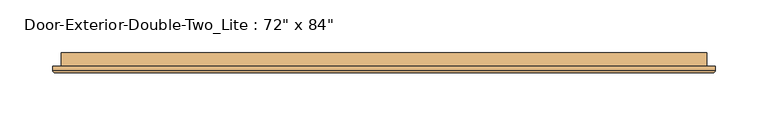
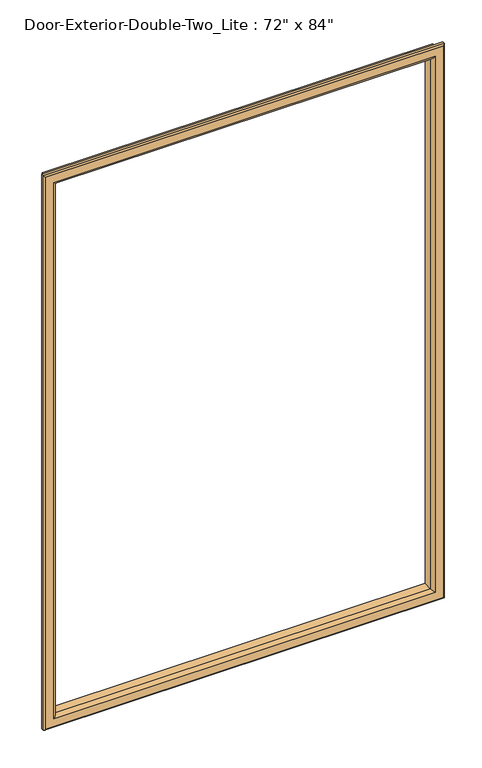
"""IFC4 building model written with IfcOpenShell, lengths in millimetres: door geometry."""

from ifc_helpers import new_model, si_unit, frame, origin, place, context, project, spatial, ellipse_curve, source, transform, mapped, element, save
from ifc_brep_helpers import plane_surface, cylinder_surface, advanced_brep


def door_d0d74375(model_context):
    return source(origin(), model_context, "Body", "AdvancedBrep", [
        advanced_brep(
        [(-762.0, 36.5125, 1117.6), (-762.0, 23.8125, 1117.6), (-762.0, 23.8125, 2016.125), (-762.0, 36.5125, 2016.125), (-750.0, 22.8125, 1129.6), (-750.0, 36.5125, 1129.6), (-750.0, 36.5125, 2004.125), (-750.0, 22.8125, 2004.125), (-755.0, 17.8125, 1124.6), (-755.0, 17.8125, 2009.125), (-770.0, 19.8125, 1109.6), (-768.0, 17.8125, 1111.6), (-768.0, 17.8125, 2022.125), (-770.0, 19.8125, 2024.125), (-770.0, 23.8125, 1109.6), (-770.0, 23.8125, 2024.125), (-152.4, 23.8125, 2016.125), (-152.4, 36.5125, 2016.125), (-164.4, 36.5125, 2004.125), (-164.4, 22.8125, 2004.125), (-159.4, 17.8125, 2009.125), (-146.4, 17.8125, 2022.125), (-144.4, 19.8125, 2024.125), (-144.4, 23.8125, 2024.125), (-152.4, 23.8125, 1117.6), (-152.4, 36.5125, 1117.6), (-164.4, 36.5125, 1129.6), (-164.4, 22.8125, 1129.6), (-159.4, 17.8125, 1124.6), (-146.4, 17.8125, 1111.6), (-144.4, 19.8125, 1109.6), (-144.4, 23.8125, 1109.6)],
        [
            (0, 1),
            (1, 2),
            (2, 3),
            (3, 0),
            (4, 5),
            (5, 6),
            (6, 7),
            (7, 4),
            (8, 4, ellipse_curve(frame((-755.0, 22.8125, 1124.6), z_axis=(-0.7071067811865475, 0.0, 0.7071067811865475), x_axis=(-0.7071067811865474, 0.0, -0.7071067811865476)), 7.0710678, 5.0)),
            (7, 9, ellipse_curve(frame((-755.0, 22.8125, 2009.125), z_axis=(-0.7071067811865475, 0.0, -0.7071067811865475), x_axis=(0.7071067811865474, 0.0, -0.7071067811865476)), 7.0710678, 5.0)),
            (9, 8),
            (10, 11, ellipse_curve(frame((-768.0, 19.8125, 1111.6), z_axis=(-0.7071067811865475, 0.0, 0.7071067811865475), x_axis=(-0.7071067811865474, 0.0, -0.7071067811865476)), 2.8284271, 2.0)),
            (11, 12),
            (12, 13, ellipse_curve(frame((-768.0, 19.8125, 2022.125), z_axis=(-0.7071067811865475, 0.0, -0.7071067811865475), x_axis=(0.7071067811865474, 0.0, -0.7071067811865476)), 2.8284271, 2.0)),
            (13, 10),
            (14, 10),
            (13, 15),
            (15, 14),
            (2, 16),
            (16, 17),
            (17, 3),
            (6, 18),
            (18, 19),
            (19, 7),
            (19, 20, ellipse_curve(frame((-159.4, 22.8125, 2009.125), z_axis=(-0.7071067811865475, 0.0, 0.7071067811865475), x_axis=(-0.7071067811865476, 0.0, -0.7071067811865474)), 7.0710678, 5.0)),
            (20, 9),
            (12, 21),
            (21, 22, ellipse_curve(frame((-146.4, 19.8125, 2022.125), z_axis=(-0.7071067811865475, 0.0, 0.7071067811865475), x_axis=(-0.7071067811865476, 0.0, -0.7071067811865474)), 2.8284271, 2.0)),
            (22, 13),
            (22, 23),
            (23, 15),
            (16, 24),
            (24, 25),
            (25, 17),
            (18, 26),
            (26, 27),
            (27, 19),
            (27, 28, ellipse_curve(frame((-159.4, 22.8125, 1124.6), z_axis=(0.7071067811865475, 0.0, 0.7071067811865475), x_axis=(-0.7071067811865474, 0.0, 0.7071067811865476)), 7.0710678, 5.0)),
            (28, 20),
            (21, 29),
            (29, 30, ellipse_curve(frame((-146.4, 19.8125, 1111.6), z_axis=(0.7071067811865475, 0.0, 0.7071067811865475), x_axis=(-0.7071067811865474, 0.0, 0.7071067811865476)), 2.8284271, 2.0)),
            (30, 22),
            (30, 31),
            (31, 23),
            (31, 14),
            (1, 24),
            (0, 25),
            (5, 26),
            (4, 27),
            (8, 28),
            (11, 29),
            (10, 30),
        ],
        [
            plane_surface(frame((-762.0, 23.8125, 1117.6), z_axis=(-1.0, 0.0, 0.0), x_axis=(0.0, 0.0, 1.0))),
            plane_surface(frame((-750.0, 36.5125, 1129.6), z_axis=(1.0, 0.0, 0.0), x_axis=(0.0, 0.0, 1.0))),
            cylinder_surface(frame((-755.0, 22.8125, 1117.6), z_axis=(0.0, 0.0, -1.0), x_axis=(-1.0, 0.0, 0.0)), 5.0),
            cylinder_surface(frame((-768.0, 19.8125, 1117.6), z_axis=(0.0, 0.0, -1.0), x_axis=(-1.0, 0.0, 0.0)), 2.0),
            plane_surface(frame((-770.0, 19.8125, 1109.6), z_axis=(-1.0, 0.0, 0.0), x_axis=(0.0, 0.0, 1.0))),
            plane_surface(frame((-762.0, 23.8125, 2016.125), z_axis=(0.0, 0.0, 1.0), x_axis=(1.0, 0.0, 0.0))),
            plane_surface(frame((-750.0, 36.5125, 2004.125), z_axis=(0.0, 0.0, -1.0), x_axis=(1.0, 0.0, 0.0))),
            cylinder_surface(frame((-762.0, 22.8125, 2009.125), z_axis=(-1.0, 0.0, 0.0), x_axis=(0.0, 0.0, 1.0)), 5.0),
            cylinder_surface(frame((-762.0, 19.8125, 2022.125), z_axis=(-1.0, 0.0, 0.0), x_axis=(0.0, 0.0, 1.0)), 2.0),
            plane_surface(frame((-770.0, 19.8125, 2024.125), z_axis=(0.0, 0.0, 1.0), x_axis=(1.0, 0.0, 0.0))),
            plane_surface(frame((-152.4, 23.8125, 2016.125), z_axis=(1.0, 0.0, 0.0), x_axis=(0.0, 0.0, -1.0))),
            plane_surface(frame((-164.4, 36.5125, 2004.125), z_axis=(-1.0, 0.0, 0.0), x_axis=(0.0, 0.0, -1.0))),
            cylinder_surface(frame((-159.4, 22.8125, 2016.125), z_axis=(0.0, 0.0, 1.0), x_axis=(1.0, 0.0, 0.0)), 5.0),
            cylinder_surface(frame((-146.4, 19.8125, 2016.125), z_axis=(0.0, 0.0, 1.0), x_axis=(1.0, 0.0, 0.0)), 2.0),
            plane_surface(frame((-144.4, 19.8125, 2024.125), z_axis=(1.0, 0.0, 0.0), x_axis=(0.0, 0.0, -1.0))),
            plane_surface(frame((-144.4, 23.8125, 1109.6), z_axis=(0.0, 1.0, 0.0), x_axis=(-1.0, 0.0, 0.0))),
            plane_surface(frame((-152.4, 23.8125, 1117.6), z_axis=(0.0, 0.0, -1.0), x_axis=(-1.0, 0.0, 0.0))),
            plane_surface(frame((-152.4, 36.5125, 1117.6), z_axis=(0.0, 1.0, 0.0), x_axis=(-1.0, 0.0, 0.0))),
            plane_surface(frame((-164.4, 36.5125, 1129.6), z_axis=(0.0, 0.0, 1.0), x_axis=(-1.0, 0.0, 0.0))),
            cylinder_surface(frame((-152.4, 22.8125, 1124.6), z_axis=(1.0, 0.0, 0.0), x_axis=(0.0, 0.0, -1.0)), 5.0),
            plane_surface(frame((-159.4, 17.8125, 1124.6), z_axis=(0.0, -1.0, 0.0), x_axis=(-1.0, 0.0, 0.0))),
            cylinder_surface(frame((-152.4, 19.8125, 1111.6), z_axis=(1.0, 0.0, 0.0), x_axis=(0.0, 0.0, -1.0)), 2.0),
            plane_surface(frame((-144.4, 19.8125, 1109.6), z_axis=(0.0, 0.0, -1.0), x_axis=(-1.0, 0.0, 0.0))),
        ],
        [
            (0, [[1, 2, 3, 4]]),
            (1, [[5, 6, 7, 8]]),
            (2, [[9, -8, 10, 11]]),
            (3, [[12, 13, 14, 15]]),
            (4, [[16, -15, 17, 18]]),
            (5, [[-3, 19, 20, 21]]),
            (6, [[-7, 22, 23, 24]]),
            (7, [[-10, -24, 25, 26]]),
            (8, [[-14, 27, 28, 29]]),
            (9, [[-17, -29, 30, 31]]),
            (10, [[-20, 32, 33, 34]]),
            (11, [[-23, 35, 36, 37]]),
            (12, [[-25, -37, 38, 39]]),
            (13, [[-28, 40, 41, 42]]),
            (14, [[-30, -42, 43, 44]]),
            (15, [[-31, -44, 45, -18], [46, -32, -19, -2]]),
            (16, [[-33, -46, -1, 47]]),
            (17, [[-21, -34, -47, -4], [48, -35, -22, -6]]),
            (18, [[-36, -48, -5, 49]]),
            (19, [[-38, -49, -9, 50]]),
            (20, [[51, -40, -27, -13], [-26, -39, -50, -11]]),
            (21, [[-41, -51, -12, 52]]),
            (22, [[-43, -52, -16, -45]]),
        ],
    ),
    ])


if __name__ == "__main__":
    model = new_model("IFC4")
    model_context = context("Model", 3, world=origin())
    ifc_project = project(units=[si_unit("LENGTHUNIT", "METRE", prefix="MILLI")], contexts=[model_context])
    site = spatial("IfcSite", under=ifc_project)
    building = spatial("IfcBuilding", under=site)
    placement = place(None, origin())
    door_shape = door_d0d74375(model_context)
    element("IfcDoor", 1, ObjectType="Door-Exterior-Double-Two_Lite : 72\" x 84\"", at=placement, inside=building, context=model_context, shape_type="MappedRepresentation", body=[
        mapped(door_shape, transform((0.0, 0.0, 0.0), x_axis=(1.0, 0.0, 0.0), y_axis=(0.0, 1.0, 0.0), z_axis=(0.0, 0.0, 1.0))),
    ])
    save(model, "model.ifc")

# Revit data of these elements
# Type "Door-Exterior-Double-Two_Lite : 72\" x 84\""
#   Type Mark = "20"
#   Assembly Code = "B2030100"
#   Analytic Construction = "Metal frame, double glass door"
#   Top Rail = 0' - 4 5/8"
#   Threshold Length [instance default] = 6' - 4"
#   Threshold Offset [instance default] = 0' - 0 1/2"
#   Thickness = 0' - 1 3/4"
#   Thermal Resistance (R) = 1.3794 (h·ft²·°F)/BTU
#   Swing Angle [instance default] = 90.00°
#   Strike Height = 3' - 4"
#   Stiles = 0' - 6"
#   SinglePanelWidth = 3' - 0"
#   Rough Width [instance default] = 6' - 4"
#   Rough Height [instance default] = 7' - 4"
#   MFOpeningHeight [instance default] = 0' - 4"
#   MFOpeningWidth [instance default] = 0' - 4"
#   Lock Rail = 0' - 8"
#   Inset Calculate [instance default] = 0' - 4"
#   Masonry Inset [instance default] = 0' - 1"
#   Height = 7' - 0"
#   Width = 6' - 0"
#   Heat Transfer Coefficient (U) = 0.7250 BTU/(h·ft²·°F)
#   Glass Thickness = 0' - 0 3/4"
#   Masonry Frame Depth = 0' - 5 3/4"
#   Bottom Rail = 0' - 10"
#   Threshold [instance default] = yes
#   Masonry Frame [instance default] = yes
#   Function = 1
#   Dry Wall Frame [instance default] = no
#   Threshold Material = none
#   Panic Bar Material = Metal - Stainless Steel
#   Panel Material = Metal - Painted - Grey
#   Glass Stop Material = Metal - Painted - Grey
#   Frame Material = Metal - Painted - Grey
#   Exterior Pull Material = Metal - Stainless Steel
#   Visual Light Transmittance = 0
#   Solar Heat Gain Coefficient = 0
#   Wall Closure = (empty or 0)
# Element 1 (IfcDoor, "Door-Exterior-Double-Two_Lite : 72\" x 84\"")
#   Threshold Length = 6' - 0"
#   Rough Width = 6' - 2 1/2"
#   Rough Height = 7' - 1 1/4"
#   MFOpeningHeight = 0' - 1 1/4"
#   MFOpeningWidth = 0' - 2 1/2"
#   Inset Calculate = 0' - 3"
#   Masonry Frame = no
#   Dry Wall Frame = yes
#   Materials on its faces: "Metal - Painted - Grey", "Metal - Stainless Steel", "Glass"
# Materials
#   "Metal - Stainless Steel": class "Metal", colour RGB 247 247 247, transparency 0
#   "Metal - Painted - Grey": class "Paint", colour RGB 104 104 104, transparency 0, Cost = 0
#   "Glass": class "Glass", colour RGB 0 128 192, transparency 0.75, Description = "Soda Lime Glass", Cost = 0
